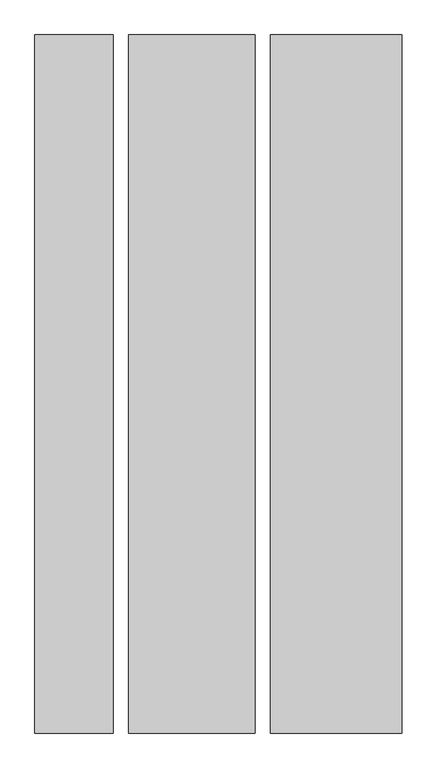
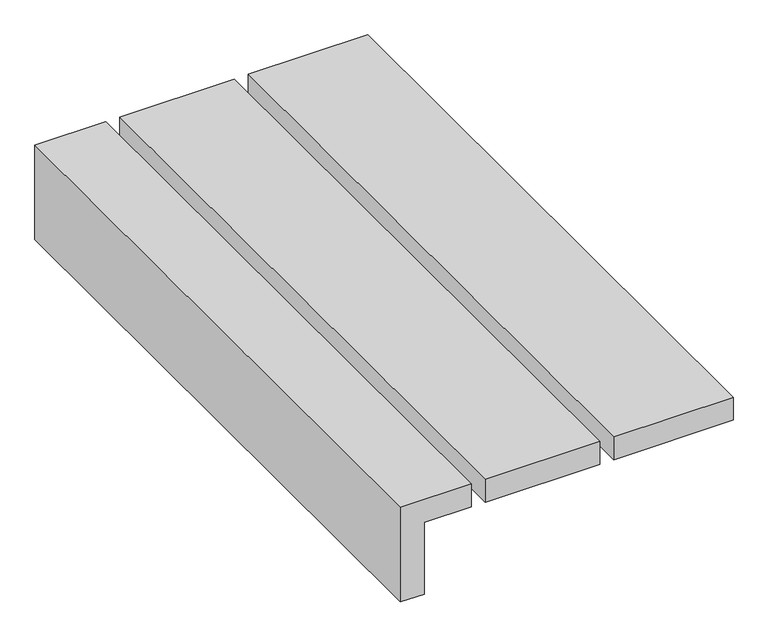
"""IFC4 building model written with IfcOpenShell, lengths in millimetres: proxy geometry, Blocking106 12412 : Blocking106 12412."""

from ifc_helpers import new_model, si_unit, frame, origin, place, context, project, spatial, polyline, outline, extrude, source, transform, mapped, element, save


def generic_models_2ceb33a1(model_context):
    return source(origin(), model_context, "Body", "SweptSolid", [
        extrude(outline(polyline([(44042.7623529, 6172.6163563), (44042.7623529, 6320.6984495), (44118.9623529, 6320.6984495), (44118.9623529, 6096.4163563), (43803.0227817, 6096.4163563), (43803.0227817, 6172.6163563), (44042.7623529, 6172.6163563)])), frame((0.0, -1052.8908936, 0.0), z_axis=(0.0, 1.0, 0.0), x_axis=(0.0, 0.0, 1.0)), (0.0, 0.0, 1.0), 2000.0),
        extrude(outline(polyline([(7149.3612048, -1052.8908936), (6771.5484495, -1052.8908936), (6771.5484495, 947.1091064), (7149.3612048, 947.1091064), (7149.3612048, -1052.8908936)])), frame((0.0, 0.0, 44042.7623529), z_axis=(0.0, 0.0, 1.0), x_axis=(1.0, 0.0, 0.0)), (0.0, 0.0, 1.0), 76.2),
        extrude(outline(polyline([(6727.0984495, -1052.8908936), (6365.1484495, -1052.8908936), (6365.1484495, 947.1091064), (6727.0984495, 947.1091064), (6727.0984495, -1052.8908936)])), frame((0.0, 0.0, 44042.7623529), z_axis=(0.0, 0.0, 1.0), x_axis=(1.0, 0.0, 0.0)), (0.0, 0.0, 1.0), 76.2),
    ])


if __name__ == "__main__":
    model = new_model("IFC4")
    model_context = context("Model", 3, world=origin())
    ifc_project = project(units=[si_unit("LENGTHUNIT", "METRE", prefix="MILLI")], contexts=[model_context])
    site = spatial("IfcSite", under=ifc_project)
    building = spatial("IfcBuilding", under=site)
    placement = place(None, origin())
    generic_models_shape = generic_models_2ceb33a1(model_context)
    element("IfcBuildingElementProxy", 1, Name="Blocking106 12412 : Blocking106 12412", ObjectType="Blocking106 12412 : Blocking106 12412", at=placement, inside=building, context=model_context, shape_type="MappedRepresentation", body=[
        mapped(generic_models_shape, transform((0.0, 0.0, 0.0), x_axis=(1.0, 0.0, 0.0), y_axis=(0.0, 1.0, 0.0), z_axis=(0.0, 0.0, 1.0))),
    ])
    save(model, "model.ifc")

# Revit data of these elements
# Type "Blocking106 12412 : Blocking106 12412"
#   NameOverride = "Blocking106"
# Element 1 (IfcBuildingElementProxy, "Blocking106 12412 : Blocking106 12412")
#   Materials on its faces: "POLYURETHANE SPRAY FOAM UNDER ROOF SUBSTRATE (SEE T-24 ENERGY REPORT FOR R-VALUE)"
# Materials
#   "POLYURETHANE SPRAY FOAM UNDER ROOF SUBSTRATE (SEE T-24 ENERGY REPORT FOR R-VALUE)": class "Unassigned", colour RGB 210 164 194, transparency 0, Cost = 0
